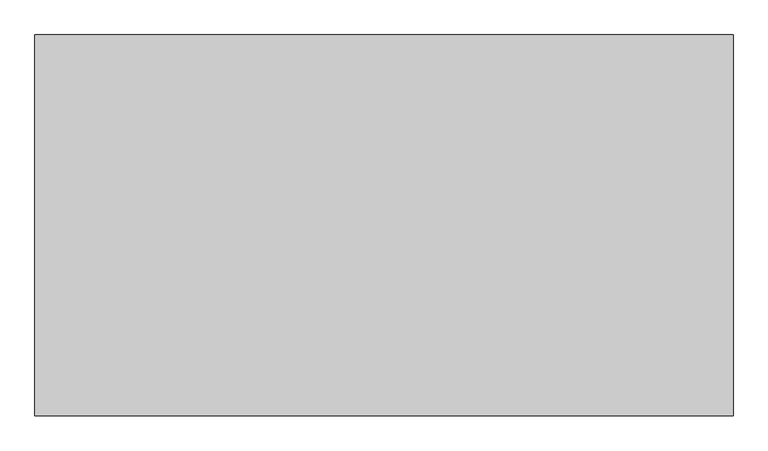
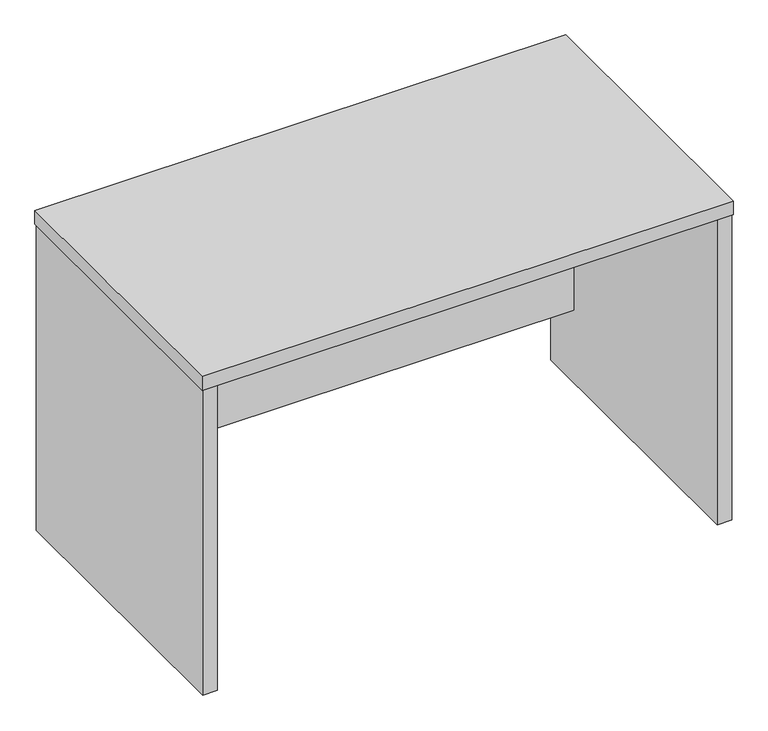
"""IFC4 building model written with IfcOpenShell, lengths in millimetres: furniture geometry, GEL-Table-一般オフィスデスク : GEL-Table-一般オフィスデスク."""

from ifc_helpers import new_model, si_unit, frame, origin, origin_with_axes, place, context, project, spatial, polyline, outline, extrude, source, transform, mapped, element, save


def furniture_45d6af98(model_context):
    return source(origin(), model_context, "Body", "SweptSolid", [
        extrude(outline(polyline([(-518.0, 217.0), (-518.0, 247.0), (518.0, 247.0), (518.0, 217.0), (-518.0, 217.0)])), frame((0.0, 0.0, 160.0), z_axis=(0.0, 0.0, 1.0), x_axis=(1.0, 0.0, 0.0)), (0.0, 0.0, 1.0), 510.0),
        extrude(outline(polyline([(518.0, -296.0), (518.0, 300.0), (548.0, 300.0), (548.0, -296.0), (518.0, -296.0)])), origin_with_axes(), (0.0, 0.0, 1.0), 670.0),
        extrude(outline(polyline([(-548.0, -296.0), (-548.0, 300.0), (-518.0, 300.0), (-518.0, -296.0), (-548.0, -296.0)])), origin_with_axes(), (0.0, 0.0, 1.0), 670.0),
        extrude(outline(polyline([(-550.0, -298.0), (-550.0, 302.0), (550.0, 302.0), (550.0, -298.0), (-550.0, -298.0)])), frame((0.0, 0.0, 670.0), z_axis=(0.0, 0.0, 1.0), x_axis=(1.0, 0.0, 0.0)), (0.0, 0.0, 1.0), 30.0),
    ])


if __name__ == "__main__":
    model = new_model("IFC4")
    model_context = context("Model", 3, world=origin())
    ifc_project = project(units=[si_unit("LENGTHUNIT", "METRE", prefix="MILLI")], contexts=[model_context])
    site = spatial("IfcSite", under=ifc_project)
    building = spatial("IfcBuilding", under=site)
    placement = place(None, origin())
    furniture_shape = furniture_45d6af98(model_context)
    element("IfcFurniture", 1, ObjectType="GEL-Table-一般オフィスデスク : GEL-Table-一般オフィスデスク", at=placement, inside=building, context=model_context, shape_type="MappedRepresentation", body=[
        mapped(furniture_shape, transform((0.0, 0.0, 0.0), x_axis=(1.0, 0.0, 0.0), y_axis=(0.0, 1.0, 0.0), z_axis=(0.0, 0.0, 1.0))),
    ])
    save(model, "model.ifc")

# Revit data of these elements
# Project information
#   プロジェクト発行日 = "発行日"
#   プロジェクト ステータス = "プロジェクト ステータス"
#   クライアント名 = "オーナ"
#   計画地住所 = "ここにアドレスを入力"
#   プロジェクト名 = "プロジェクト名"
#   プロジェクト番号 = "0001"
# Type "GEL-Table-一般オフィスデスク : GEL-Table-一般オフィスデスク"
#   GEL-Width = 1100 mm
#   GEL-Height = 700 mm
#   GEL-Depth = 600 mm
#   GEL-Material-Top = Walnut brown polished
#   GEL-Material-Support = Walnut brown polished
#   GEL-Material-Base = none
#   GEL-Material-Accent = none
#   Default Elevation = 0
# Element 1 (IfcFurniture, "GEL-Table-一般オフィスデスク : GEL-Table-一般オフィスデスク")
#   Materials on its faces: "Walnut brown polished"
# Materials
#   "Walnut brown polished": class "一般", colour RGB 103 67 45, transparency 0, Cost = 0
